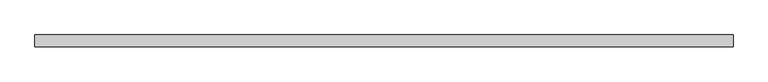
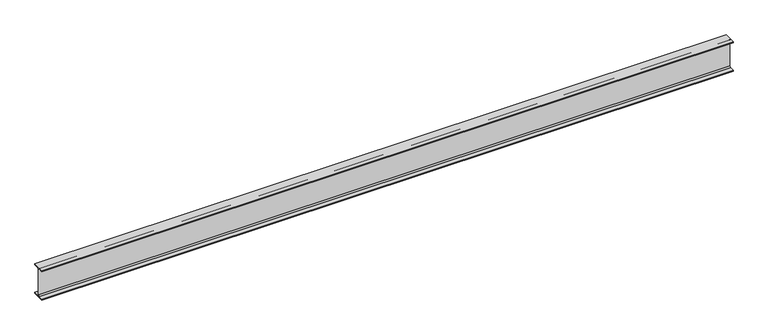
"""IFC4 building model written with IfcOpenShell, lengths in millimetres: beam geometry, Steel Framing_H_KS : H_SB_AR_S02_H-800x300x14x26_SRB1."""

from ifc_helpers import new_model, si_unit, point, frame, frame_2d, origin, place, context, project, spatial, polyline, circle_curve, trimmed, segment, composite_curve, outline, extrude, source, transform, mapped, element, save


def beam_9fd407d8(model_context):
    return source(origin(), model_context, "Body", "SweptSolid", [
        extrude(outline(composite_curve([segment(polyline([(150.0, -374.0), (150.0, -400.0), (-150.0, -400.0), (-150.0, -374.0), (-35.0, -374.0)]), True, "CONTINUOUS"), segment(trimmed(circle_curve(frame_2d((-35.0, -346.0)), 28.0), [point((-35.0, -374.0))], [point((-7.0, -346.0))], True, "CARTESIAN"), True, "CONTINUOUS"), segment(polyline([(-7.0, -346.0), (-7.0, 346.0)]), True, "CONTINUOUS"), segment(trimmed(circle_curve(frame_2d((-35.0, 346.0)), 28.0), [point((-7.0, 346.0))], [point((-35.0, 374.0))], True, "CARTESIAN"), True, "CONTINUOUS"), segment(polyline([(-35.0, 374.0), (-150.0, 374.0), (-150.0, 400.0), (150.0, 400.0), (150.0, 374.0), (35.0, 374.0)]), True, "CONTINUOUS"), segment(trimmed(circle_curve(frame_2d((35.0, 346.0)), 28.0), [point((35.0, 374.0))], [point((7.0, 346.0))], True, "CARTESIAN"), True, "CONTINUOUS"), segment(polyline([(7.0, 346.0), (7.0, -346.0)]), True, "CONTINUOUS"), segment(trimmed(circle_curve(frame_2d((35.0, -346.0)), 28.0), [point((7.0, -346.0))], [point((35.0, -374.0))], True, "CARTESIAN"), True, "CONTINUOUS"), segment(polyline([(35.0, -374.0), (150.0, -374.0)]), True, "CONTINUOUS")], self_intersect=False)), frame((-8837.3, 0.0, 0.0), z_axis=(1.0, 0.0, 0.0), x_axis=(0.0, 1.0, 0.0)), (0.0, 0.0, 1.0), 17749.6),
    ])


if __name__ == "__main__":
    model = new_model("IFC4")
    model_context = context("Model", 3, world=origin())
    ifc_project = project(units=[si_unit("LENGTHUNIT", "METRE", prefix="MILLI")], contexts=[model_context])
    site = spatial("IfcSite", under=ifc_project)
    building = spatial("IfcBuilding", under=site)
    placement = place(None, origin())
    beam_shape = beam_9fd407d8(model_context)
    element("IfcBeam", 1, ObjectType="Steel Framing_H_KS : H_SB_AR_S02_H-800x300x14x26_SRB1", at=placement, inside=building, context=model_context, shape_type="MappedRepresentation", body=[
        mapped(beam_shape, transform((0.0, 0.0, 0.0), x_axis=(1.0, 0.0, 0.0), y_axis=(0.0, 1.0, 0.0), z_axis=(0.0, 0.0, 1.0))),
    ])
    save(model, "model.ifc")

# Revit data of these elements
# Type "Steel Framing_H_KS : H_SB_AR_S02_H-800x300x14x26_SRB1"
#   Type Comments = "MAIN"
#   Type Mark = "SRB1"
#   H_SectionID = "H-800x300x14x26"
#   H_Ratio for Additional Steel Plate = 0.2
#   Width = 30.0 cm
#   Web Thickness = 1.4 cm
#   Web Fillet = 2.8 cm
#   Warping Constant = 17500000.0 cm⁶
#   Torsional Moment of Inertia = 422.315 cm⁴
#   Section Area = 267.4 cm²
#   Plastic Modulus weak axis = 1220.0 cm³
#   Plastic Modulus strong axis = 8240.0 cm³
#   Perimeter = 2.72 m²/m
#   Nominal Weight = 210.00 kgf/m
#   Moment of Inertia weak axis = 11700.00 cm⁴
#   Moment of Inertia strong axis = 292000.00 cm⁴
#   Height = 80.0 cm
#   Flange Thickness = 2.6 cm
#   Elastic Modulus weak axis = 782.0 cm³
#   Elastic Modulus strong axis = 7290.0 cm³
#   Centroid Vertical = 40.0 cm
#   Centroid Horizontal = 15.0 cm
#   Bolt Spacing = 8.89 cm
#   Length [instance default] = 1500 mm
#   Structural Material [instance default] = Steel, 45-345
#   Section Name Key = ""
#   Assembly Code = ""
# Element 1 (IfcBeam, "Steel Framing_H_KS : H_SB_AR_S02_H-800x300x14x26_SRB1")
#   Materials on its faces: "Steel, 45-345"
# Materials
#   "Steel, 45-345": class "Metal", colour RGB 189 187 185, transparency 0, Description = "Steel 345 MPa", Cost = 0
